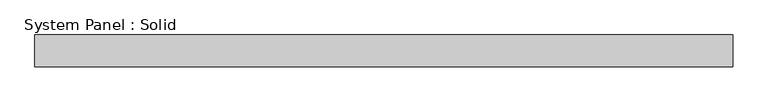
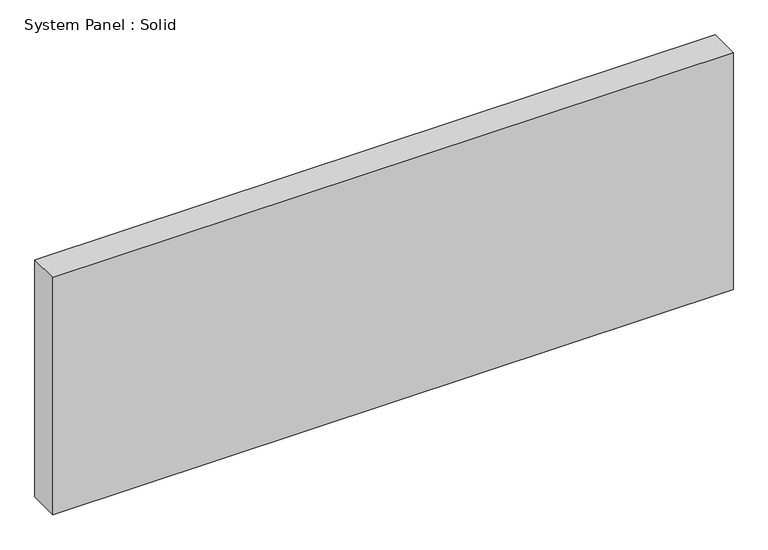
"""IFC4 building model written with IfcOpenShell, lengths in millimetres: plate geometry, System Panel : Solid."""

import ifcopenshell
import ifcopenshell.guid

model = None  # the IFC model being written
_history = None  # IfcOwnerHistory: only IFC2X3 demands one
_inside = {}  # id of a spatial element -> (the spatial element, [elements in it])
_under = {}  # id of a project, library or spatial element -> (it, [spatial elements below it])
_declared = {}  # id of a project -> (the project, [libraries it declares])
_typed = {}  # id of a type object -> (the type object, [elements of that type])
_made_of = {}  # id of a material, layer set ... -> (it, [elements and type objects made of it])


def new_model(schema):
    """Start an empty IFC model of exactly this schema.

    Asked for "IFC4X3", IfcOpenShell would pick the latest addendum, in which some entities
    have other attributes; the version numbers below select the first issue.
    IFC2X3 requires an IfcOwnerHistory on every rooted entity: one is made here for all.
    """
    global model, _history
    if schema == "IFC4X3":
        model = ifcopenshell.file(schema_version=(4, 3, 0, 0))
    else:
        model = ifcopenshell.file(schema=schema)
    _inside.clear()
    _under.clear()
    _declared.clear()
    _typed.clear()
    _made_of.clear()
    _history = None
    if model.schema == "IFC2X3":
        org = make("IfcOrganization", Name="unknown")
        user = make(
            "IfcPersonAndOrganization",
            ThePerson=make("IfcPerson", FamilyName="unknown"),
            TheOrganization=org,
        )
        app = make(
            "IfcApplication",
            ApplicationDeveloper=org,
            Version="unknown",
            ApplicationFullName="unknown",
            ApplicationIdentifier="unknown",
        )
        _history = make(
            "IfcOwnerHistory",
            OwningUser=user,
            OwningApplication=app,
            ChangeAction="ADDED",
            CreationDate=0,
        )
    return model


def make(cls, **values):
    """One entity of the class cls with the attributes given. An attribute that is None is left unset."""
    return model.create_entity(
        cls, **{name: value for name, value in values.items() if value is not None}
    )


def rooted(cls, **values):
    """An entity with a GlobalId (a new one), such as an element, a storey or a relation."""
    return make(cls, GlobalId=ifcopenshell.guid.new(), OwnerHistory=_history, **values)


def si_unit(unit_type, name, prefix=None):
    """IfcSIUnit, for example si_unit("LENGTHUNIT", "METRE", prefix="MILLI")."""
    return make("IfcSIUnit", UnitType=unit_type, Prefix=prefix, Name=name)


def assignment(units):
    """IfcUnitAssignment: the units of a project."""
    return None if units is None else make("IfcUnitAssignment", Units=units)


def point(xyz):
    """IfcCartesianPoint."""
    return None if xyz is None else make("IfcCartesianPoint", Coordinates=xyz)


def direction(xyz):
    """IfcDirection."""
    return None if xyz is None else make("IfcDirection", DirectionRatios=xyz)


def frame(location, z_axis=None, x_axis=None):
    """IfcAxis2Placement3D, a coordinate frame: its origin and axes. An axis left out is left unset."""
    return make(
        "IfcAxis2Placement3D",
        Location=point(location),
        Axis=direction(z_axis),
        RefDirection=direction(x_axis),
    )


def origin():
    """The frame at (0, 0, 0) with its axes left unset."""
    return frame((0.0, 0.0, 0.0))


def origin_with_axes():
    """The frame at (0, 0, 0) with the z axis (0, 0, 1) and the x axis (1, 0, 0) written out."""
    return frame((0.0, 0.0, 0.0), z_axis=(0.0, 0.0, 1.0), x_axis=(1.0, 0.0, 0.0))


def place(relative_to, where):
    """IfcLocalPlacement: puts the frame where relative to a parent placement (None: the world)."""
    return make(
        "IfcLocalPlacement", PlacementRelTo=relative_to, RelativePlacement=where
    )


def context(
    kind, dimensions, precision=None, world=None, true_north=None, identifier=None
):
    """IfcGeometricRepresentationContext, for example the 3D "Model" context."""
    return make(
        "IfcGeometricRepresentationContext",
        ContextIdentifier=identifier,
        ContextType=kind,
        CoordinateSpaceDimension=dimensions,
        Precision=precision,
        WorldCoordinateSystem=world,
        TrueNorth=true_north,
    )


def project(units=None, contexts=None):
    """IfcProject with its units and contexts."""
    return rooted(
        "IfcProject",
        Name="project",
        RepresentationContexts=contexts,
        UnitsInContext=assignment(units),
    )


def spatial(cls, under=None, at=None, **own):
    """A site, building, storey or space (cls), placed at a placement, below another one or the project."""
    s = rooted(cls, ObjectPlacement=at, **own)
    if under is not None:
        _under.setdefault(under.id(), (under, []))[1].append(s)
    return s


def polyline(points):
    """IfcPolyline through the points."""
    return make("IfcPolyline", Points=[point(p) for p in points])


def outline(outer, holes=None, kind="AREA"):
    """IfcArbitraryClosedProfileDef: a profile drawn as a closed curve; with holes, ...WithVoids."""
    if holes is None:
        return make("IfcArbitraryClosedProfileDef", ProfileType=kind, OuterCurve=outer)
    return make(
        "IfcArbitraryProfileDefWithVoids",
        ProfileType=kind,
        OuterCurve=outer,
        InnerCurves=holes,
    )


def extrude(swept, where, along, depth):
    """IfcExtrudedAreaSolid: the profile swept, set in the frame where, extruded along a direction by depth."""
    return make(
        "IfcExtrudedAreaSolid",
        SweptArea=swept,
        Position=where,
        ExtrudedDirection=direction(along),
        Depth=depth,
    )


def shape(context_of_items, identifier, shape_type, items):
    """IfcShapeRepresentation: the items that make up one representation, for example the "Body"."""
    return make(
        "IfcShapeRepresentation",
        ContextOfItems=context_of_items,
        RepresentationIdentifier=identifier,
        RepresentationType=shape_type,
        Items=items,
    )


def source(mapping_origin, context_of_items, identifier, shape_type, items):
    """IfcRepresentationMap: a shape defined once, which mapped items show again and again."""
    return make(
        "IfcRepresentationMap",
        MappingOrigin=mapping_origin,
        MappedRepresentation=shape(context_of_items, identifier, shape_type, items),
    )


def transform(
    local_origin,
    x_axis=None,
    y_axis=None,
    z_axis=None,
    scale=None,
    scale2=None,
    scale3=None,
    uniform=True,
):
    """IfcCartesianTransformationOperator3D, or its non-uniform kind. x_axis, y_axis, z_axis: its Axis1, 2, 3."""
    if uniform:
        return make(
            "IfcCartesianTransformationOperator3D",
            Axis1=direction(x_axis),
            Axis2=direction(y_axis),
            LocalOrigin=point(local_origin),
            Scale=scale,
            Axis3=direction(z_axis),
        )
    return make(
        "IfcCartesianTransformationOperator3DnonUniform",
        Axis1=direction(x_axis),
        Axis2=direction(y_axis),
        LocalOrigin=point(local_origin),
        Scale=scale,
        Axis3=direction(z_axis),
        Scale2=scale2,
        Scale3=scale3,
    )


def mapped(mapping_source, mapping_target):
    """IfcMappedItem: shows the shape of a source again, moved by a transform."""
    return make(
        "IfcMappedItem", MappingSource=mapping_source, MappingTarget=mapping_target
    )


def made_of(thing, what):
    """Note that an element or type object is made of a material, layer set ...; save() writes the relation."""
    if what is not None:
        _made_of.setdefault(what.id(), (what, []))[1].append(thing)
    return thing


def element(
    cls,
    number,
    at=None,
    inside=None,
    cuts=None,
    type_object=None,
    material=None,
    context=None,
    identifier="Body",
    shape_type=None,
    held_by="IfcProductDefinitionShape",
    body=None,
    shapes=None,
    **own,
):
    """One element of the class cls, such as IfcWall. Its Tag is "e" and its number.

    at: its placement. inside: the storey or other place that contains it. cuts: it is an
    opening in that element (IfcRelVoidsElement). A single representation is given by context,
    identifier, shape_type and body (its items); several are given by shapes. held_by: the class
    of the entity that holds the representations. save() writes the other relations.
    """
    e = rooted(cls, Tag="e%d" % number, ObjectPlacement=at, **own)
    if body is not None:
        shapes = [shape(context, identifier, shape_type, body)]
    if shapes is not None:
        e.Representation = make(held_by, Representations=shapes)
    if inside is not None:
        _inside.setdefault(inside.id(), (inside, []))[1].append(e)
    if cuts is not None:
        rooted(
            "IfcRelVoidsElement", RelatingBuildingElement=cuts, RelatedOpeningElement=e
        )
    if type_object is not None:
        _typed.setdefault(type_object.id(), (type_object, []))[1].append(e)
    return made_of(e, material)


def aggregate(whole, parts):
    """IfcRelAggregates: a whole, such as a stair, and the parts it consists of."""
    return rooted("IfcRelAggregates", RelatingObject=whole, RelatedObjects=parts)


def save(model, path):
    """Write the relations noted so far, then the file.

    IfcRelAggregates (storeys below a building ...), IfcRelContainedInSpatialStructure (elements
    in a storey), IfcRelDefinesByType, IfcRelAssociatesMaterial and IfcRelDeclares: one each for
    every whole, place, type object, material and project.
    """
    for whole, parts in _under.values():
        aggregate(whole, parts)
    for where, things in _inside.values():
        rooted(
            "IfcRelContainedInSpatialStructure",
            RelatedElements=things,
            RelatingStructure=where,
        )
    for kind, things in _typed.values():
        rooted("IfcRelDefinesByType", RelatedObjects=things, RelatingType=kind)
    for what, things in _made_of.values():
        rooted("IfcRelAssociatesMaterial", RelatedObjects=things, RelatingMaterial=what)
    for by, libraries in _declared.values():
        rooted("IfcRelDeclares", RelatingContext=by, RelatedDefinitions=libraries)
    model.write(path)


def system_panel_solid_21827ae2(model_context):
    return source(origin(), model_context, "Body", "SweptSolid", [
        extrude(outline(polyline([(697.4416668, -19.05), (-697.4416668, -19.05), (-697.4416668, 44.45), (697.4416668, 44.45), (697.4416668, -19.05)])), origin_with_axes(), (0.0, 0.0, 1.0), 514.35),
    ])


if __name__ == "__main__":
    model = new_model("IFC4")
    model_context = context("Model", 3, world=origin())
    ifc_project = project(units=[si_unit("LENGTHUNIT", "METRE", prefix="MILLI")], contexts=[model_context])
    site = spatial("IfcSite", under=ifc_project)
    building = spatial("IfcBuilding", under=site)
    placement = place(None, origin())
    system_panel_solid_shape = system_panel_solid_21827ae2(model_context)
    element("IfcPlate", 1, ObjectType="System Panel : Solid", at=placement, inside=building, context=model_context, shape_type="MappedRepresentation", body=[
        mapped(system_panel_solid_shape, transform((0.0, 0.0, 0.0), x_axis=(1.0, 0.0, 0.0), y_axis=(0.0, 1.0, 0.0), z_axis=(0.0, 0.0, 1.0))),
    ])
    save(model, "model.ifc")

# Revit data of these elements
# Type "System Panel : Solid"
#   Construction Type Id = "MDOOR"
#   Analytic Construction = "Metal"
#   Visual Light Transmittance = 0
#   Solar Heat Gain Coefficient = 0
#   Heat Transfer Coefficient (U) = 0.651978 BTU/(h·ft²·°F)
#   Define Thermal Properties by = 1
# Element 1 (IfcPlate, "System Panel : Solid")
#   Materials on its faces: "Default"
# Materials
#   "Default": class "Miscellaneous", colour RGB 127 127 127, transparency 0, Cost = 0
